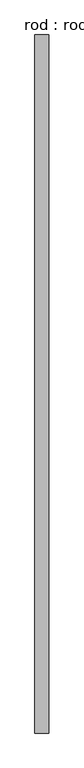
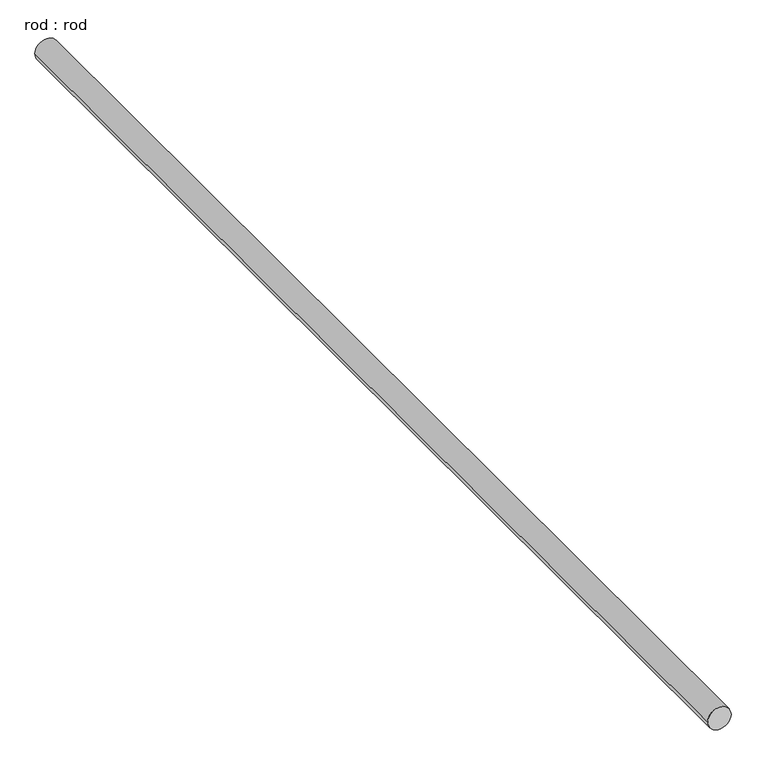
"""IFC4 building model written with IfcOpenShell, lengths in millimetres: proxy geometry, rod : rod."""

from ifc_helpers import new_model, si_unit, point, frame, frame_2d, origin, place, context, project, spatial, circle_curve, trimmed, segment, composite_curve, outline, extrude, source, transform, mapped, element, save


def rod_rod_463a696d(model_context):
    return source(origin(), model_context, "Body", "SweptSolid", [
        extrude(outline(composite_curve([segment(trimmed(circle_curve(frame_2d((0.0108462, 0.0)), 200.0), [point((0.0108462, 200.0))], [point((0.0108462, -200.0))], False, "CARTESIAN"), True, "CONTINUOUS"), segment(trimmed(circle_curve(frame_2d((0.0108462, 0.0)), 200.0), [point((0.0108462, -200.0))], [point((0.0108462, 200.0))], False, "CARTESIAN"), True, "CONTINUOUS")], self_intersect=False)), frame((0.0, -5871.5570989, 0.0), z_axis=(0.0, 1.0, 0.0), x_axis=(0.0, 0.0, 1.0)), (0.0, 0.0, 1.0), 19928.5714286),
    ])


if __name__ == "__main__":
    model = new_model("IFC4")
    model_context = context("Model", 3, world=origin())
    ifc_project = project(units=[si_unit("LENGTHUNIT", "METRE", prefix="MILLI")], contexts=[model_context])
    site = spatial("IfcSite", under=ifc_project)
    building = spatial("IfcBuilding", under=site)
    placement = place(None, origin())
    rod_rod_shape = rod_rod_463a696d(model_context)
    element("IfcBuildingElementProxy", 1, Name="rod : rod", ObjectType="rod : rod", at=placement, inside=building, context=model_context, shape_type="MappedRepresentation", body=[
        mapped(rod_rod_shape, transform((0.0, 0.0, 0.0), x_axis=(1.0, 0.0, 0.0), y_axis=(0.0, 1.0, 0.0), z_axis=(0.0, 0.0, 1.0))),
    ])
    save(model, "model.ifc")

# Revit data of these elements
# Type "rod : rod"
#   Default Elevation = 0
